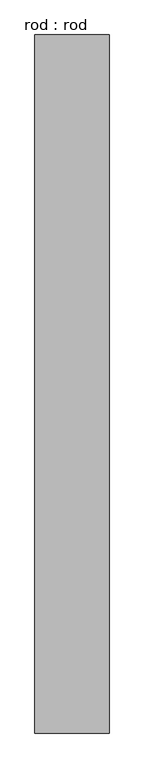
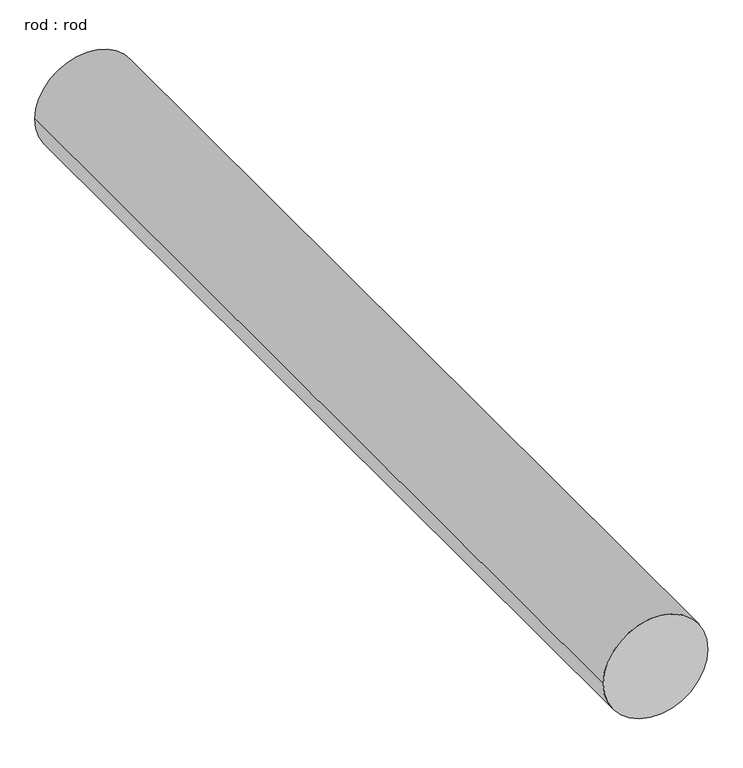
"""IFC4 building model written with IfcOpenShell, lengths in millimetres: proxy geometry, rod : rod."""

from ifc_helpers import new_model, si_unit, point, frame, frame_2d, origin, place, context, project, spatial, circle_curve, trimmed, segment, composite_curve, outline, extrude, source, transform, mapped, element, save


def rod_rod_8c728755(model_context):
    return source(origin(), model_context, "Body", "SweptSolid", [
        extrude(outline(composite_curve([segment(trimmed(circle_curve(frame_2d((0.0108462, 0.0)), 200.0), [point((0.0108462, 200.0))], [point((0.0108462, -200.0))], False, "CARTESIAN"), True, "CONTINUOUS"), segment(trimmed(circle_curve(frame_2d((0.0108462, 0.0)), 200.0), [point((0.0108462, -200.0))], [point((0.0108462, 200.0))], False, "CARTESIAN"), True, "CONTINUOUS")], self_intersect=False)), frame((0.0, 2208.9838608, 0.0), z_axis=(0.0, 1.0, 0.0), x_axis=(0.0, 0.0, 1.0)), (0.0, 0.0, 1.0), 3767.489509),
    ])


if __name__ == "__main__":
    model = new_model("IFC4")
    model_context = context("Model", 3, world=origin())
    ifc_project = project(units=[si_unit("LENGTHUNIT", "METRE", prefix="MILLI")], contexts=[model_context])
    site = spatial("IfcSite", under=ifc_project)
    building = spatial("IfcBuilding", under=site)
    placement = place(None, origin())
    rod_rod_shape = rod_rod_8c728755(model_context)
    element("IfcBuildingElementProxy", 1, Name="rod : rod", ObjectType="rod : rod", at=placement, inside=building, context=model_context, shape_type="MappedRepresentation", body=[
        mapped(rod_rod_shape, transform((0.0, 0.0, 0.0), x_axis=(1.0, 0.0, 0.0), y_axis=(0.0, 1.0, 0.0), z_axis=(0.0, 0.0, 1.0))),
    ])
    save(model, "model.ifc")

# Revit data of these elements
# Type "rod : rod"
#   Default Elevation = 0
